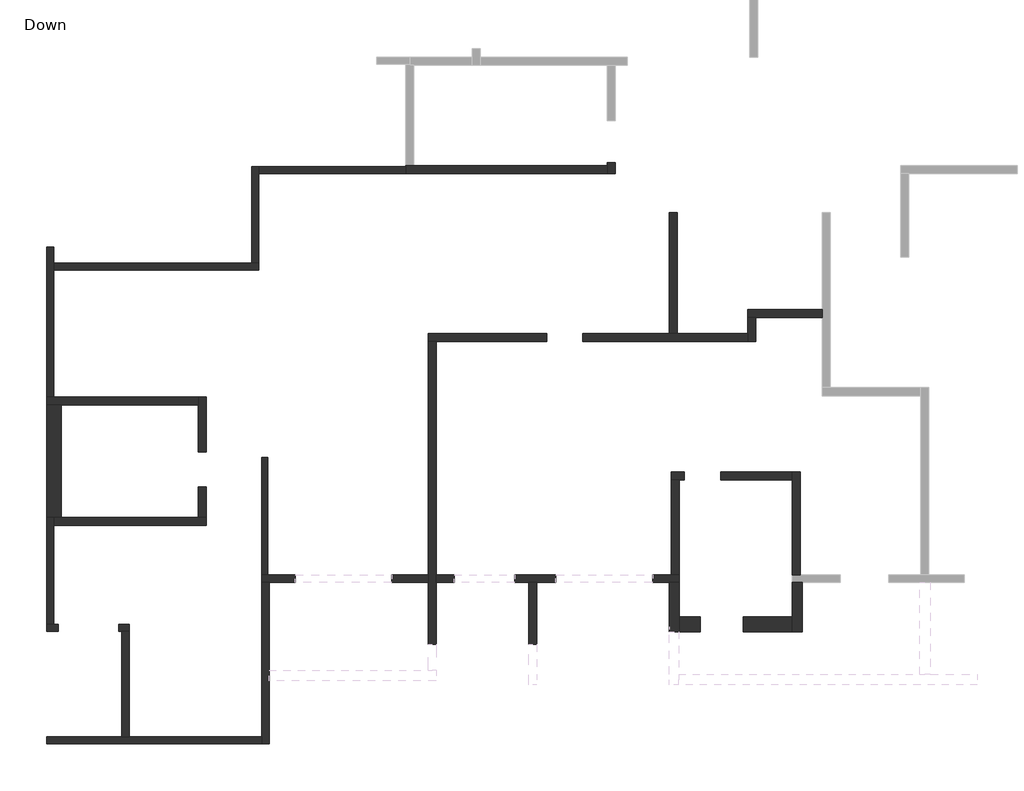
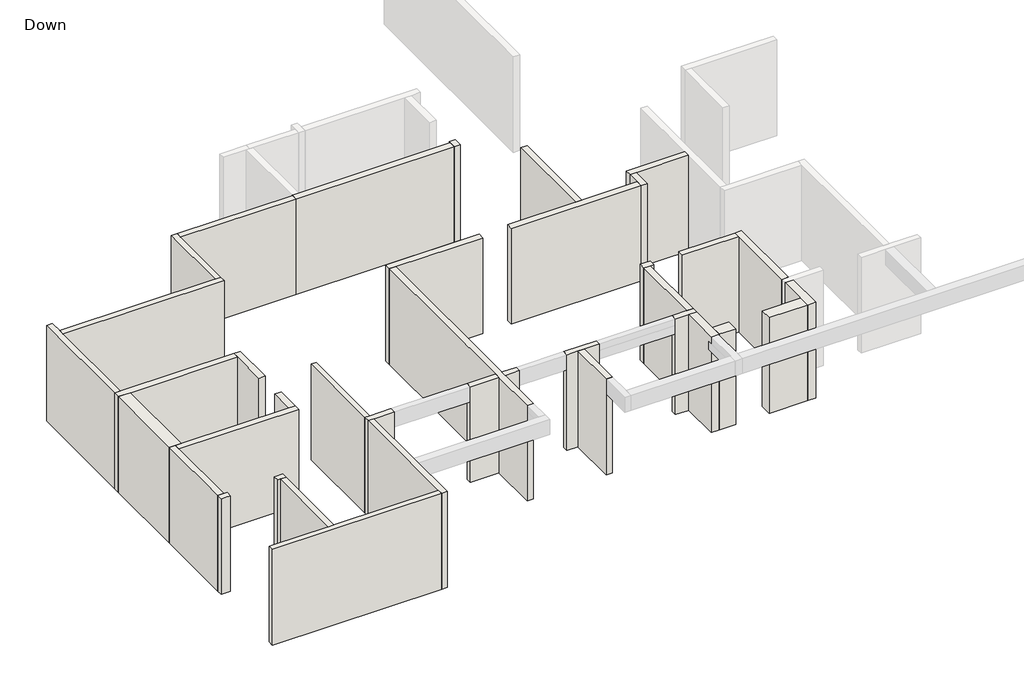
# One storey, part 1 of 3: 38 walls.
"""IFC4 building model written with IfcOpenShell, lengths in millimetres."""

from ifc_helpers import new_model, si_unit, origin, place, context, project, spatial, faceted_brep, element, save

model = new_model("IFC4")

# Units and contexts
model_context = context("Model", 3, world=origin())
ifc_project = project(units=[si_unit("LENGTHUNIT", "METRE", prefix="MILLI")], contexts=[model_context])

# Site, building, storey
site = spatial("IfcSite", under=ifc_project)
building = spatial("IfcBuilding", under=site)
storey = spatial("IfcBuildingStorey", under=building, Name="Down", Elevation=0.0)

# Walls
placement = place(None, origin())
element("IfcWall", 1, ObjectType="15", at=placement, inside=storey, context=model_context, shape_type="Brep", body=[
    faceted_brep([(-13197.6689839, -11344.051338, 0.0), (-13197.6689839, -8414.0928317, 0.0), (-13197.6689839, -8414.0928317, 3000.0), (-13197.6689839, -8414.0928317, 3200.0), (-13197.6689839, -11344.051338, 3200.0), (-13197.6689839, -11344.051338, 3000.0), (-13347.6689839, -11344.051338, 0.0), (-13347.6689839, -11344.051338, 3200.0), (-13347.6689839, -8414.0928317, 3200.0), (-13347.6689839, -8414.0928317, 3000.0), (-13347.6689839, -8414.0928317, 0.0)], [[[0, 1, 2, 3, 4, 5]], [[6, 7, 8, 9, 10]], [[1, 0, 6, 10]], [[3, 2, 1, 10, 9, 8]], [[4, 3, 8, 7]], [[0, 5, 4, 7, 6]]]),
])
element("IfcWall", 2, ObjectType="18", at=placement, inside=storey, context=model_context, shape_type="Brep", body=[
    faceted_brep([(-9216.2167018, -11344.051338, 0.0), (-10116.2830918, -11344.051338, 0.0), (-10116.2830918, -11344.051338, 2700.0), (-10116.2830918, -11344.051338, 3200.0), (-9216.2167018, -11344.051338, 3200.0), (-9216.2167018, -11344.051338, 3000.0), (-9216.2167018, -11524.051338, 0.0), (-9216.2167018, -11524.051338, 2980.0), (-9216.2167018, -11524.051338, 3200.0), (-10116.2830918, -11524.051338, 3200.0), (-10116.2830918, -11524.051338, 2700.0), (-10116.2830918, -11524.051338, 0.0)], [[[0, 1, 2, 3, 4, 5]], [[6, 7, 8, 9, 10, 11]], [[1, 0, 6, 11]], [[3, 2, 1, 11, 10, 9]], [[4, 3, 9, 8]], [[0, 5, 4, 8, 7, 6]]]),
])
element("IfcWall", 3, ObjectType="18", at=placement, inside=storey, context=model_context, shape_type="Brep", body=[
    faceted_brep([(-12517.1627599, -11344.051338, 0.0), (-13197.6689839, -11344.051338, 0.0), (-13347.6689839, -11344.051338, 0.0), (-13347.6689839, -11344.051338, 3200.0), (-13197.6689839, -11344.051338, 3200.0), (-12517.1627599, -11344.051338, 3200.0), (-12517.1627599, -11344.051338, 2700.0), (-12517.1627599, -11524.051338, 0.0), (-12517.1627599, -11524.051338, 2700.0), (-12517.1627599, -11524.051338, 3200.0), (-13167.6689839, -11524.051338, 3200.0), (-13347.6689839, -11524.051338, 3200.0), (-13347.6689839, -11524.051338, 0.0), (-13167.6689839, -11524.051338, 0.0)], [[[0, 1, 2, 3, 4, 5, 6]], [[7, 8, 9, 10, 11, 12, 13]], [[2, 1, 0, 7, 13, 12]], [[5, 4, 3, 11, 10, 9]], [[0, 6, 5, 9, 8, 7]], [[3, 2, 12, 11]]]),
])
element("IfcWall", 4, ObjectType="18", at=placement, inside=storey, context=model_context, shape_type="Brep", body=[
    faceted_brep([(-13347.6689839, -11524.051338, 0.0), (-13347.6689839, -15365.0637861, 0.0), (-13347.6689839, -15545.0637861, 0.0), (-13347.6689839, -15545.0637861, 3200.0), (-13347.6689839, -15365.0637861, 3200.0), (-13347.6689839, -11524.051338, 3200.0), (-13167.6689839, -11524.051338, 0.0), (-13167.6689839, -11524.051338, 2980.0), (-13167.6689839, -11524.051338, 3200.0), (-13167.6689839, -13713.3127488, 3200.0), (-13167.6689839, -15545.0637861, 3200.0), (-13167.6689839, -15545.0637861, 0.0)], [[[0, 1, 2, 3, 4, 5]], [[6, 7, 8, 9, 10, 11]], [[2, 1, 0, 6, 11]], [[5, 4, 3, 10, 9, 8]], [[0, 5, 8, 7, 6]], [[3, 2, 11, 10]]]),
])
element("IfcWall", 5, ObjectType="18", at=placement, inside=storey, context=model_context, shape_type="Brep", body=[
    faceted_brep([(-2966.3411831, -11344.051338, 0.0), (-2966.5901458, -11344.051338, 0.0), (-3166.5901458, -11344.051338, 0.0), (-3636.648237, -11344.051338, 0.0), (-3636.648237, -11344.051338, 2700.0), (-3636.648237, -11344.051338, 3200.0), (-3166.5901458, -11344.051338, 3200.0), (-2966.5901458, -11344.051338, 3200.0), (-2966.3411831, -11344.051338, 3200.0), (-2966.3411831, -11344.051338, 3000.0), (-2966.3411831, -11524.051338, 0.0), (-2966.3411831, -11524.051338, 3200.0), (-3216.3411831, -11524.051338, 3200.0), (-3636.648237, -11524.051338, 3200.0), (-3636.648237, -11524.051338, 2980.0), (-3636.648237, -11524.051338, 2700.0), (-3636.648237, -11524.051338, 0.0), (-3216.3411831, -11524.051338, 0.0), (-3636.648237, -11519.051338, 3200.0)], [[[0, 1, 2, 3, 4, 5, 6, 7, 8, 9]], [[10, 11, 12, 13, 14, 15, 16, 17]], [[3, 2, 1, 0, 10, 17, 16]], [[5, 4, 3, 16, 15, 14, 13, 18]], [[8, 7, 6, 5, 18, 13, 12, 11]], [[0, 9, 8, 11, 10]]]),
])
element("IfcWall", 6, ObjectType="18", at=placement, inside=storey, context=model_context, shape_type="Brep", body=[
    faceted_brep([(-6035.4200213, -11344.051338, 0.0), (-7066.175208, -11344.051338, 0.0), (-7066.175208, -11344.051338, 2700.0), (-7066.175208, -11344.051338, 3200.0), (-6035.4200213, -11344.051338, 3200.0), (-6035.4200213, -11344.051338, 2700.0), (-6035.4200213, -11524.051338, 0.0), (-6035.4200213, -11524.051338, 2700.0), (-6035.4200213, -11524.051338, 2980.0), (-6035.4200213, -11524.051338, 3200.0), (-6516.0175316, -11524.051338, 3200.0), (-6716.0175316, -11524.051338, 3200.0), (-7066.175208, -11524.051338, 3200.0), (-7066.175208, -11524.051338, 2700.0), (-7066.175208, -11524.051338, 0.0), (-6716.0175316, -11524.051338, 0.0), (-6516.0175316, -11524.051338, 0.0), (-6035.4200213, -11519.051338, 3200.0)], [[[0, 1, 2, 3, 4, 5]], [[6, 7, 8, 9, 10, 11, 12, 13, 14, 15, 16]], [[1, 0, 6, 16, 15, 14]], [[3, 2, 1, 14, 13, 12]], [[4, 3, 12, 11, 10, 9, 17]], [[0, 5, 4, 17, 9, 8, 7, 6]]]),
])
element("IfcWall", 7, ObjectType="18", at=placement, inside=storey, context=model_context, shape_type="Brep", body=[
    faceted_brep([(-8566.988486, -11344.051338, 0.0), (-9016.2167018, -11344.051338, 0.0), (-9016.2167018, -11344.051338, 3000.0), (-9016.2167018, -11344.051338, 3200.0), (-8566.988486, -11344.051338, 3200.0), (-8566.988486, -11344.051338, 2700.0), (-8566.988486, -11524.051338, 0.0), (-8566.988486, -11524.051338, 2700.0), (-8566.988486, -11524.051338, 3200.0), (-9016.2167018, -11524.051338, 3200.0), (-9016.2167018, -11524.051338, 0.0)], [[[0, 1, 2, 3, 4, 5]], [[6, 7, 8, 9, 10]], [[1, 0, 6, 10]], [[4, 3, 9, 8]], [[0, 5, 4, 8, 7, 6]], [[3, 2, 1, 10, 9]]]),
])
element("IfcWall", 8, ObjectType="18", at=placement, inside=storey, context=model_context, shape_type="Brep", body=[
    faceted_brep([(-13347.6689839, -15365.0637861, 0.0), (-16646.5071582, -15365.0637861, 0.0), (-16826.5071582, -15365.0637861, 0.0), (-18697.4781126, -15365.0637861, 0.0), (-18697.4781126, -15365.0637861, 3200.0), (-18561.2442958, -15365.0637861, 3200.0), (-16826.5071582, -15365.0637861, 3200.0), (-16646.5071582, -15365.0637861, 3200.0), (-13347.6689839, -15365.0637861, 3200.0), (-13347.6689839, -15365.0637861, 3000.0), (-13347.6689839, -15545.0637861, 0.0), (-13347.6689839, -15545.0637861, 3200.0), (-18697.4781126, -15545.0637861, 3200.0), (-18697.4781126, -15545.0637861, 0.0)], [[[0, 1, 2, 3, 4, 5, 6, 7, 8, 9]], [[10, 11, 12, 13]], [[3, 2, 1, 0, 10, 13]], [[4, 3, 13, 12]], [[8, 7, 6, 5, 4, 12, 11]], [[0, 9, 8, 11, 10]]]),
])
element("IfcWall", 9, ObjectType="18", at=placement, inside=storey, context=model_context, shape_type="Brep", body=[
    faceted_brep([(-16646.5071582, -15365.0637861, 0.0), (-16646.5071582, -12744.5160683, 0.0), (-16646.5071582, -12744.5160683, 3200.0), (-16646.5071582, -15365.0637861, 3200.0), (-16646.5071582, -15365.0637861, 3000.0), (-16826.5071582, -15365.0637861, 0.0), (-16826.5071582, -15365.0637861, 2980.0), (-16826.5071582, -15365.0637861, 3200.0), (-16826.5071582, -12744.5160683, 3200.0), (-16826.5071582, -12744.5160683, 2980.0), (-16826.5071582, -12744.5160683, 0.0)], [[[0, 1, 2, 3, 4]], [[5, 6, 7, 8, 9, 10]], [[1, 0, 5, 10]], [[3, 2, 8, 7]], [[2, 1, 10, 9, 8]], [[0, 4, 3, 7, 6, 5]]]),
])
element("IfcWall", 10, ObjectType="18", at=placement, inside=storey, context=model_context, shape_type="Brep", body=[
    faceted_brep([(-16646.5071582, -12564.5160683, 0.0), (-16907.8847516, -12564.5160683, 0.0), (-16907.8847516, -12564.5160683, 3000.0), (-16907.8847516, -12564.5160683, 3200.0), (-16646.5071582, -12564.5160683, 3200.0), (-16646.5071582, -12564.5160683, 3000.0), (-16646.5071582, -12744.5160683, 0.0), (-16646.5071582, -12744.5160683, 3200.0), (-16826.5071582, -12744.5160683, 3200.0), (-16907.8847516, -12744.5160683, 3200.0), (-16907.8847516, -12744.5160683, 3000.0), (-16907.8847516, -12744.5160683, 0.0), (-16826.5071582, -12744.5160683, 0.0)], [[[0, 1, 2, 3, 4, 5]], [[6, 7, 8, 9, 10, 11, 12]], [[1, 0, 6, 12, 11]], [[3, 2, 1, 11, 10, 9]], [[4, 3, 9, 8, 7]], [[0, 5, 4, 7, 6]]]),
])
element("IfcWall", 11, ObjectType="18", at=placement, inside=storey, context=model_context, shape_type="Brep", body=[
    faceted_brep([(-18406.5901458, -12564.5160683, 0.0), (-18517.4781126, -12564.5160683, 0.0), (-18697.4781126, -12564.5160683, 0.0), (-18697.4781126, -12564.5160683, 3200.0), (-18517.4781126, -12564.5160683, 3200.0), (-18406.5901458, -12564.5160683, 3200.0), (-18406.5901458, -12564.5160683, 3000.0), (-18406.5901458, -12744.5160683, 0.0), (-18406.5901458, -12744.5160683, 3000.0), (-18406.5901458, -12744.5160683, 3200.0), (-18561.2442958, -12744.5160683, 3200.0), (-18697.4781126, -12744.5160683, 3200.0), (-18697.4781126, -12744.5160683, 0.0)], [[[0, 1, 2, 3, 4, 5, 6]], [[7, 8, 9, 10, 11, 12]], [[2, 1, 0, 7, 12]], [[5, 4, 3, 11, 10, 9]], [[0, 6, 5, 9, 8, 7]], [[3, 2, 12, 11]]]),
])
element("IfcWall", 12, ObjectType="18", at=placement, inside=storey, context=model_context, shape_type="Brep", body=[
    faceted_brep([(-18517.4781126, -12564.5160683, 0.0), (-18517.4781126, -10113.0471886, 0.0), (-18517.4781126, -9913.0471886, 0.0), (-18517.4781126, -9913.0471886, 3200.0), (-18517.4781126, -10113.0471886, 3200.0), (-18517.4781126, -12564.5160683, 3200.0), (-18517.4781126, -12564.5160683, 3000.0), (-18697.4781126, -12564.5160683, 0.0), (-18697.4781126, -12564.5160683, 3200.0), (-18697.4781126, -9913.0471886, 3200.0), (-18697.4781126, -9913.0471886, 0.0)], [[[0, 1, 2, 3, 4, 5, 6]], [[7, 8, 9, 10]], [[2, 1, 0, 7, 10]], [[5, 4, 3, 9, 8]], [[0, 6, 5, 8, 7]], [[3, 2, 10, 9]]]),
])
element("IfcWall", 13, ObjectType="18", at=placement, inside=storey, context=model_context, shape_type="Brep", body=[
    faceted_brep([(-18517.4781126, -6913.2795537, 0.0), (-18517.4781126, -3764.1011305, 0.0), (-18517.4781126, -3584.1011305, 0.0), (-18517.4781126, -3184.4330807, 0.0), (-18517.4781126, -3184.4330807, 3200.0), (-18517.4781126, -3584.1011305, 3200.0), (-18517.4781126, -3764.1011305, 3200.0), (-18517.4781126, -6913.2795537, 3200.0), (-18517.4781126, -6913.2795537, 3000.0), (-18697.4781126, -6913.2795537, 0.0), (-18697.4781126, -6913.2795537, 3200.0), (-18697.4781126, -3184.4330807, 3200.0), (-18697.4781126, -3184.4330807, 0.0)], [[[0, 1, 2, 3, 4, 5, 6, 7, 8]], [[9, 10, 11, 12]], [[3, 2, 1, 0, 9, 12]], [[4, 3, 12, 11]], [[7, 6, 5, 4, 11, 10]], [[0, 8, 7, 10, 9]]]),
])
element("IfcWall", 14, ObjectType="18", at=placement, inside=storey, context=model_context, shape_type="Brep", body=[
    faceted_brep([(-18517.4781126, -3764.1011305, 0.0), (-13417.2291499, -3764.1011305, 0.0), (-13417.2291499, -3764.1011305, 3000.0), (-13417.2291499, -3764.1011305, 3200.0), (-18517.4781126, -3764.1011305, 3200.0), (-18517.4781126, -3764.1011305, 3000.0), (-18517.4781126, -3584.1011305, 0.0), (-18517.4781126, -3584.1011305, 3200.0), (-13597.2291499, -3584.1011305, 3200.0), (-13417.2291499, -3584.1011305, 3200.0), (-13417.2291499, -3584.1011305, 0.0), (-13597.2291499, -3584.1011305, 0.0)], [[[0, 1, 2, 3, 4, 5]], [[6, 7, 8, 9, 10, 11]], [[1, 0, 6, 11, 10]], [[4, 3, 9, 8, 7]], [[0, 5, 4, 7, 6]], [[3, 2, 1, 10, 9]]]),
])
element("IfcWall", 15, ObjectType="18", at=placement, inside=storey, context=model_context, shape_type="Brep", body=[
    faceted_brep([(-13417.2291499, -3584.1011305, 0.0), (-13417.2291499, -1364.051338, 0.0), (-13417.2291499, -1184.051338, 0.0), (-13417.2291499, -1184.051338, 3200.0), (-13417.2291499, -1364.051338, 3200.0), (-13417.2291499, -3584.1011305, 3200.0), (-13597.2291499, -3584.1011305, 0.0), (-13597.2291499, -3584.1011305, 3200.0), (-13597.2291499, -1184.051338, 3200.0), (-13597.2291499, -1184.051338, 0.0)], [[[0, 1, 2, 3, 4, 5]], [[6, 7, 8, 9]], [[2, 1, 0, 6, 9]], [[5, 4, 3, 8, 7]], [[0, 5, 7, 6]], [[3, 2, 9, 8]]]),
])
element("IfcWall", 16, ObjectType="18", at=placement, inside=storey, context=model_context, shape_type="Brep", body=[
    faceted_brep([(-13417.2291499, -1364.051338, 0.0), (-9767.2291499, -1364.051338, 0.0), (-9767.2291499, -1364.051338, 3200.0), (-13417.2291499, -1364.051338, 3200.0), (-13417.2291499, -1364.051338, 3000.0), (-13417.2291499, -1184.051338, 0.0), (-13417.2291499, -1184.051338, 3200.0), (-9767.2291499, -1184.051338, 3200.0), (-9767.2291499, -1184.051338, 0.0)], [[[0, 1, 2, 3, 4]], [[5, 6, 7, 8]], [[1, 0, 5, 8]], [[2, 1, 8, 7]], [[3, 2, 7, 6]], [[0, 4, 3, 6, 5]]]),
])
element("IfcWall", 17, ObjectType="20", at=placement, inside=storey, context=model_context, shape_type="Brep", body=[
    faceted_brep([(35.0364103, -11344.051338, 0.0), (35.0364103, -8782.9724998, 0.0), (35.0364103, -8782.9724998, 3000.0), (35.0364103, -8782.9724998, 3200.0), (35.0364103, -11344.051338, 3200.0), (35.0364103, -11344.051338, 3000.0), (-164.9635897, -11344.051338, 0.0), (-164.9635897, -11344.051338, 3200.0), (-164.9635897, -8982.9724998, 3200.0), (-164.9635897, -8782.9724998, 3200.0), (-164.9635897, -8782.9724998, 0.0), (-164.9635897, -8982.9724998, 0.0)], [[[0, 1, 2, 3, 4, 5]], [[6, 7, 8, 9, 10, 11]], [[1, 0, 6, 11, 10]], [[4, 3, 9, 8, 7]], [[0, 5, 4, 7, 6]], [[3, 2, 1, 10, 9]]]),
])
element("IfcWall", 18, ObjectType="20", at=placement, inside=storey, context=model_context, shape_type="Brep", body=[
    faceted_brep([(-164.9635897, -8782.9724998, 0.0), (-1944.0175316, -8782.9724998, 0.0), (-1944.0175316, -8782.9724998, 3000.0), (-1944.0175316, -8782.9724998, 3200.0), (-164.9635897, -8782.9724998, 3200.0), (-164.9635897, -8982.9724998, 0.0), (-164.9635897, -8982.9724998, 3000.0), (-164.9635897, -8982.9724998, 3200.0), (-1944.0175316, -8982.9724998, 3200.0), (-1944.0175316, -8982.9724998, 3000.0), (-1944.0175316, -8982.9724998, 0.0)], [[[0, 1, 2, 3, 4]], [[5, 6, 7, 8, 9, 10]], [[1, 0, 5, 10]], [[3, 2, 1, 10, 9, 8]], [[4, 3, 8, 7]], [[0, 4, 7, 6, 5]]]),
])
element("IfcWall", 19, ObjectType="20", at=placement, inside=storey, context=model_context, shape_type="Brep", body=[
    faceted_brep([(-2850.4075731, -8782.9724998, 0.0), (-3166.5901458, -8782.9724998, 0.0), (-3166.5901458, -8782.9724998, 3000.0), (-3166.5901458, -8782.9724998, 3200.0), (-2850.4075731, -8782.9724998, 3200.0), (-2850.4075731, -8782.9724998, 3000.0), (-2850.4075731, -8982.9724998, 0.0), (-2850.4075731, -8982.9724998, 3000.0), (-2850.4075731, -8982.9724998, 3200.0), (-2966.5901458, -8982.9724998, 3200.0), (-3166.5901458, -8982.9724998, 3200.0), (-3166.5901458, -8982.9724998, 0.0), (-2966.5901458, -8982.9724998, 0.0)], [[[0, 1, 2, 3, 4, 5]], [[6, 7, 8, 9, 10, 11, 12]], [[1, 0, 6, 12, 11]], [[4, 3, 10, 9, 8]], [[0, 5, 4, 8, 7, 6]], [[3, 2, 1, 11, 10]]]),
])
element("IfcWall", 20, ObjectType="20", at=placement, inside=storey, context=model_context, shape_type="Brep", body=[
    faceted_brep([(-3166.5901458, -8982.9724998, 0.0), (-3166.5901458, -11344.051338, 0.0), (-3166.5901458, -11344.051338, 3000.0), (-3166.5901458, -11344.051338, 3200.0), (-3166.5901458, -8982.9724998, 3200.0), (-2966.5901458, -8982.9724998, 0.0), (-2966.5901458, -8982.9724998, 3000.0), (-2966.5901458, -8982.9724998, 3200.0), (-2966.5901458, -11344.051338, 3200.0), (-2966.5901458, -11344.051338, 3000.0), (-2966.5901458, -11344.051338, 0.0)], [[[0, 1, 2, 3, 4]], [[5, 6, 7, 8, 9, 10]], [[1, 0, 5, 10]], [[4, 3, 8, 7]], [[0, 4, 7, 6, 5]], [[3, 2, 1, 10, 9, 8]]]),
])
element("IfcWall", 21, ObjectType="20", at=placement, inside=storey, context=model_context, shape_type="Brep", body=[
    faceted_brep([(583.3351654, -4733.7276865, 0.0), (-1265.2789424, -4733.7276865, 0.0), (-1265.2789424, -4733.7276865, 3200.0), (583.3351654, -4733.7276865, 3200.0), (583.3351654, -4933.7276865, 0.0), (583.3351654, -4933.7276865, 3000.0), (583.3351654, -4933.7276865, 3200.0), (-1065.2789424, -4933.7276865, 3200.0), (-1265.2789424, -4933.7276865, 3200.0), (-1265.2789424, -4933.7276865, 0.0), (-1065.2789424, -4933.7276865, 0.0)], [[[0, 1, 2, 3]], [[4, 5, 6, 7, 8, 9, 10]], [[1, 0, 4, 10, 9]], [[3, 2, 8, 7, 6]], [[0, 3, 6, 5, 4]], [[2, 1, 9, 8]]]),
])
element("IfcWall", 22, ObjectType="20", at=placement, inside=storey, context=model_context, shape_type="Brep", body=[
    faceted_brep([(-1265.2789424, -4933.7276865, 0.0), (-1265.2789424, -5334.7235371, 0.0), (-1265.2789424, -5534.7235371, 0.0), (-1265.2789424, -5534.7235371, 3200.0), (-1265.2789424, -5334.7235371, 3200.0), (-1265.2789424, -4933.7276865, 3200.0), (-1065.2789424, -4933.7276865, 0.0), (-1065.2789424, -4933.7276865, 3000.0), (-1065.2789424, -4933.7276865, 3200.0), (-1065.2789424, -5534.7235371, 3200.0), (-1065.2789424, -5534.7235371, 3000.0), (-1065.2789424, -5534.7235371, 0.0)], [[[0, 1, 2, 3, 4, 5]], [[6, 7, 8, 9, 10, 11]], [[2, 1, 0, 6, 11]], [[5, 4, 3, 9, 8]], [[0, 5, 8, 7, 6]], [[3, 2, 11, 10, 9]]]),
])
element("IfcWall", 23, ObjectType="20", at=placement, inside=storey, context=model_context, shape_type="Brep", body=[
    faceted_brep([(-1265.2789424, -5334.7235371, 0.0), (-3016.9303947, -5334.7235371, 0.0), (-3216.9303947, -5334.7235371, 0.0), (-5367.2208511, -5334.7235371, 0.0), (-5367.2208511, -5334.7235371, 3000.0), (-5367.2208511, -5334.7235371, 3200.0), (-3216.9303947, -5334.7235371, 3200.0), (-3016.9303947, -5334.7235371, 3200.0), (-1265.2789424, -5334.7235371, 3200.0), (-1265.2789424, -5534.7235371, 0.0), (-1265.2789424, -5534.7235371, 3200.0), (-5367.2208511, -5534.7235371, 3200.0), (-5367.2208511, -5534.7235371, 3000.0), (-5367.2208511, -5534.7235371, 0.0)], [[[0, 1, 2, 3, 4, 5, 6, 7, 8]], [[9, 10, 11, 12, 13]], [[3, 2, 1, 0, 9, 13]], [[5, 4, 3, 13, 12, 11]], [[8, 7, 6, 5, 11, 10]], [[0, 8, 10, 9]]]),
])
element("IfcWall", 24, ObjectType="20", at=placement, inside=storey, context=model_context, shape_type="Brep", body=[
    faceted_brep([(-6267.2872412, -5334.7235371, 0.0), (-9216.2167018, -5334.7235371, 0.0), (-9216.2167018, -5334.7235371, 3000.0), (-9216.2167018, -5334.7235371, 3200.0), (-6267.2872412, -5334.7235371, 3200.0), (-6267.2872412, -5334.7235371, 3000.0), (-6267.2872412, -5534.7235371, 0.0), (-6267.2872412, -5534.7235371, 3000.0), (-6267.2872412, -5534.7235371, 3200.0), (-9016.2167018, -5534.7235371, 3200.0), (-9216.2167018, -5534.7235371, 3200.0), (-9216.2167018, -5534.7235371, 0.0), (-9016.2167018, -5534.7235371, 0.0)], [[[0, 1, 2, 3, 4, 5]], [[6, 7, 8, 9, 10, 11, 12]], [[1, 0, 6, 12, 11]], [[4, 3, 10, 9, 8]], [[0, 5, 4, 8, 7, 6]], [[3, 2, 1, 11, 10]]]),
])
element("IfcWall", 25, ObjectType="20", at=placement, inside=storey, context=model_context, shape_type="Brep", body=[
    faceted_brep([(-3216.9303947, -2332.8480185, 0.0), (-3216.9303947, -5334.7235371, 0.0), (-3216.9303947, -5334.7235371, 3000.0), (-3216.9303947, -5334.7235371, 3200.0), (-3216.9303947, -2332.8480185, 3200.0), (-3216.9303947, -2332.8480185, 3000.0), (-3016.9303947, -2332.8480185, 0.0), (-3016.9303947, -2332.8480185, 3200.0), (-3016.9303947, -5334.7235371, 3200.0), (-3016.9303947, -5334.7235371, 0.0)], [[[0, 1, 2, 3, 4, 5]], [[6, 7, 8, 9]], [[1, 0, 6, 9]], [[4, 3, 8, 7]], [[0, 5, 4, 7, 6]], [[3, 2, 1, 9, 8]]]),
])
element("IfcWall", 26, ObjectType="20", at=placement, inside=storey, context=model_context, shape_type="Brep", body=[
    faceted_brep([(-9216.2167018, -5534.7235371, 0.0), (-9216.2167018, -11344.051338, 0.0), (-9216.2167018, -11524.051338, 0.0), (-9216.2167018, -13068.3003006, 0.0), (-9216.2167018, -13068.3003006, 2700.0), (-9216.2167018, -13068.3003006, 2980.0), (-9216.2167018, -13068.3003006, 3200.0), (-9216.2167018, -11524.051338, 3200.0), (-9216.2167018, -11344.051338, 3200.0), (-9216.2167018, -5534.7235371, 3200.0), (-9016.2167018, -5534.7235371, 0.0), (-9016.2167018, -5534.7235371, 3000.0), (-9016.2167018, -5534.7235371, 3200.0), (-9016.2167018, -11344.051338, 3200.0), (-9016.2167018, -11524.051338, 3200.0), (-9016.2167018, -13068.3003006, 3200.0), (-9016.2167018, -13068.3003006, 2700.0), (-9016.2167018, -13068.3003006, 0.0), (-9016.2167018, -11524.051338, 0.0), (-9016.2167018, -11344.051338, 0.0), (-9211.2167018, -13068.3003006, 3200.0)], [[[0, 1, 2, 3, 4, 5, 6, 7, 8, 9]], [[10, 11, 12, 13, 14, 15, 16, 17, 18, 19]], [[3, 2, 1, 0, 10, 19, 18, 17]], [[6, 5, 4, 3, 17, 16, 15, 20]], [[9, 8, 7, 6, 20, 15, 14, 13, 12]], [[0, 9, 12, 11, 10]]]),
])
element("IfcWall", 27, ObjectType="20", at=placement, inside=storey, context=model_context, shape_type="Brep", body=[
    faceted_brep([(-6716.0175316, -11524.051338, 0.0), (-6716.0175316, -13068.3003006, 0.0), (-6716.0175316, -13068.3003006, 2700.0), (-6716.0175316, -13068.3003006, 3200.0), (-6716.0175316, -11524.051338, 3200.0), (-6516.0175316, -11524.051338, 0.0), (-6516.0175316, -11524.051338, 2980.0), (-6516.0175316, -11524.051338, 3200.0), (-6516.0175316, -13068.3003006, 3200.0), (-6516.0175316, -13068.3003006, 2700.0), (-6516.0175316, -13068.3003006, 0.0)], [[[0, 1, 2, 3, 4]], [[5, 6, 7, 8, 9, 10]], [[1, 0, 5, 10]], [[3, 2, 1, 10, 9, 8]], [[4, 3, 8, 7]], [[0, 4, 7, 6, 5]]]),
])
element("IfcWall", 28, ObjectType="20", at=placement, inside=storey, context=model_context, shape_type="Brep", body=[
    faceted_brep([(-18517.4781126, -10113.0471886, 0.0), (-14726.2250005, -10113.0471886, 0.0), (-14726.2250005, -10113.0471886, 3000.0), (-14726.2250005, -10113.0471886, 3200.0), (-18517.4781126, -10113.0471886, 3200.0), (-18517.4781126, -10113.0471886, 3000.0), (-18517.4781126, -9913.0471886, 0.0), (-18517.4781126, -9913.0471886, 3200.0), (-18327.4781126, -9913.0471886, 3200.0), (-14926.2250005, -9913.0471886, 3200.0), (-14726.2250005, -9913.0471886, 3200.0), (-14726.2250005, -9913.0471886, 0.0), (-14926.2250005, -9913.0471886, 0.0), (-18327.4781126, -9913.0471886, 0.0)], [[[0, 1, 2, 3, 4, 5]], [[6, 7, 8, 9, 10, 11, 12, 13]], [[1, 0, 6, 13, 12, 11]], [[4, 3, 10, 9, 8, 7]], [[0, 5, 4, 7, 6]], [[3, 2, 1, 11, 10]]]),
])
element("IfcWall", 29, ObjectType="20", at=placement, inside=storey, context=model_context, shape_type="Brep", body=[
    faceted_brep([(-14726.2250005, -9913.0471886, 0.0), (-14726.2250005, -9149.744284, 0.0), (-14726.2250005, -9149.744284, 3000.0), (-14726.2250005, -9149.744284, 3200.0), (-14726.2250005, -9913.0471886, 3200.0), (-14926.2250005, -9913.0471886, 0.0), (-14926.2250005, -9913.0471886, 3000.0), (-14926.2250005, -9913.0471886, 3200.0), (-14926.2250005, -9149.744284, 3200.0), (-14926.2250005, -9149.744284, 3000.0), (-14926.2250005, -9149.744284, 0.0)], [[[0, 1, 2, 3, 4]], [[5, 6, 7, 8, 9, 10]], [[1, 0, 5, 10]], [[3, 2, 1, 10, 9, 8]], [[4, 3, 8, 7]], [[0, 4, 7, 6, 5]]]),
])
element("IfcWall", 30, ObjectType="20", at=placement, inside=storey, context=model_context, shape_type="Brep", body=[
    faceted_brep([(-14726.2250005, -8279.1882674, 0.0), (-14726.2250005, -6913.2795537, 0.0), (-14726.2250005, -6913.2795537, 3000.0), (-14726.2250005, -6913.2795537, 3200.0), (-14726.2250005, -8279.1882674, 3200.0), (-14726.2250005, -8279.1882674, 3000.0), (-14926.2250005, -8279.1882674, 0.0), (-14926.2250005, -8279.1882674, 3000.0), (-14926.2250005, -8279.1882674, 3200.0), (-14926.2250005, -7113.2795537, 3200.0), (-14926.2250005, -6913.2795537, 3200.0), (-14926.2250005, -6913.2795537, 0.0), (-14926.2250005, -7113.2795537, 0.0)], [[[0, 1, 2, 3, 4, 5]], [[6, 7, 8, 9, 10, 11, 12]], [[1, 0, 6, 12, 11]], [[4, 3, 10, 9, 8]], [[0, 5, 4, 8, 7, 6]], [[3, 2, 1, 11, 10]]]),
])
element("IfcWall", 31, ObjectType="20", at=placement, inside=storey, context=model_context, shape_type="Brep", body=[
    faceted_brep([(-14926.2250005, -6913.2795537, 0.0), (-18517.4781126, -6913.2795537, 0.0), (-18697.4781126, -6913.2795537, 0.0), (-18697.4781126, -6913.2795537, 3200.0), (-18517.4781126, -6913.2795537, 3200.0), (-14926.2250005, -6913.2795537, 3200.0), (-14926.2250005, -7113.2795537, 0.0), (-14926.2250005, -7113.2795537, 3000.0), (-14926.2250005, -7113.2795537, 3200.0), (-18327.4781126, -7113.2795537, 3200.0), (-18697.4781126, -7113.2795537, 3200.0), (-18697.4781126, -7113.2795537, 0.0), (-18327.4781126, -7113.2795537, 0.0)], [[[0, 1, 2, 3, 4, 5]], [[6, 7, 8, 9, 10, 11, 12]], [[2, 1, 0, 6, 12, 11]], [[5, 4, 3, 10, 9, 8]], [[0, 5, 8, 7, 6]], [[3, 2, 11, 10]]]),
])
element("IfcWall", 32, ObjectType="20", at=placement, inside=storey, context=model_context, shape_type="Brep", body=[
    faceted_brep([(-9767.2291499, -1364.051338, 0.0), (-4766.2250005, -1364.051338, 0.0), (-4766.2250005, -1364.051338, 3200.0), (-9767.2291499, -1364.051338, 3200.0), (-9767.2291499, -1164.051338, 0.0), (-9767.2291499, -1164.051338, 3200.0), (-9766.1254155, -1164.051338, 3200.0), (-9566.1254155, -1164.051338, 3200.0), (-4766.2250005, -1164.051338, 3200.0), (-4766.2250005, -1164.051338, 0.0), (-9566.1254155, -1164.051338, 0.0), (-9766.1254155, -1164.051338, 0.0), (-9767.2291499, -1184.051338, 0.0), (-9767.2291499, -1184.051338, 3200.0)], [[[0, 1, 2, 3]], [[4, 5, 6, 7, 8, 9, 10, 11]], [[1, 0, 12, 4, 11, 10, 9]], [[3, 2, 8, 7, 6, 5, 13]], [[0, 3, 13, 5, 4, 12]], [[2, 1, 9, 8]]]),
])
element("IfcWall", 33, ObjectType="20", at=placement, inside=storey, context=model_context, shape_type="Brep", body=[
    faceted_brep([(-4566.2250005, -1364.051338, 0.0), (-4566.2250005, -1089.1965662, 0.0), (-4566.2250005, -1089.1965662, 3200.0), (-4566.2250005, -1364.051338, 3200.0), (-4566.2250005, -1364.051338, 3000.0), (-4766.2250005, -1364.051338, 0.0), (-4766.2250005, -1364.051338, 3200.0), (-4766.2250005, -1164.051338, 3200.0), (-4766.2250005, -1089.1965662, 3200.0), (-4766.2250005, -1089.1965662, 0.0), (-4766.2250005, -1164.051338, 0.0)], [[[0, 1, 2, 3, 4]], [[5, 6, 7, 8, 9, 10]], [[1, 0, 5, 10, 9]], [[2, 1, 9, 8]], [[3, 2, 8, 7, 6]], [[0, 4, 3, 6, 5]]]),
])
element("IfcWall", 34, ObjectType="25", at=placement, inside=storey, context=model_context, shape_type="Brep", body=[
    faceted_brep([(-3216.3411831, -11524.051338, 0.0), (-3216.3411831, -12754.2256118, 0.0), (-3216.3411831, -12754.2256118, 2700.0), (-3216.3411831, -12754.2256118, 2980.0), (-3216.3411831, -12754.2256118, 3200.0), (-3216.3411831, -11524.051338, 3200.0), (-3216.3411831, -11524.051338, 2980.0), (-2966.3411831, -11524.051338, 0.0), (-2966.3411831, -11524.051338, 3200.0), (-2966.3411831, -12384.2256118, 3200.0), (-2966.3411831, -12754.2256118, 3200.0), (-2966.3411831, -12754.2256118, 0.0), (-2966.3411831, -12384.2256118, 0.0), (-3211.3411831, -12754.2256118, 3200.0), (-2990.4458666, -12754.2256118, 3200.0)], [[[0, 1, 2, 3, 4, 5, 6]], [[7, 8, 9, 10, 11, 12]], [[1, 0, 7, 12, 11]], [[5, 4, 13, 14, 10, 9, 8]], [[0, 6, 5, 8, 7]], [[4, 3, 2, 1, 11, 10, 14, 13]]]),
])
element("IfcWall", 35, ObjectType="25", at=placement, inside=storey, context=model_context, shape_type="Brep", body=[
    faceted_brep([(-164.9635897, -11524.051338, 0.0), (-164.9635897, -12384.2256118, 0.0), (-164.9635897, -12754.2256118, 0.0), (-164.9635897, -12754.2256118, 3200.0), (-164.9635897, -12384.2256118, 3200.0), (-164.9635897, -11524.051338, 3200.0), (85.0364103, -11524.051338, 0.0), (85.0364103, -11524.051338, 3200.0), (85.0364103, -12754.2256118, 3200.0), (85.0364103, -12754.2256118, 0.0)], [[[0, 1, 2, 3, 4, 5]], [[6, 7, 8, 9]], [[2, 1, 0, 6, 9]], [[5, 4, 3, 8, 7]], [[0, 5, 7, 6]], [[3, 2, 9, 8]]]),
])
element("IfcWall", 36, ObjectType="37", at=placement, inside=storey, context=model_context, shape_type="Brep", body=[
    faceted_brep([(-2966.3411831, -12754.2256118, 0.0), (-2445.6938802, -12754.2256118, 0.0), (-2445.6938802, -12754.2256118, 3200.0), (-2966.3411831, -12754.2256118, 3200.0), (-2966.3411831, -12384.2256118, 0.0), (-2966.3411831, -12384.2256118, 3000.0), (-2966.3411831, -12384.2256118, 3200.0), (-2445.6938802, -12384.2256118, 3200.0), (-2445.6938802, -12384.2256118, 0.0)], [[[0, 1, 2, 3]], [[4, 5, 6, 7, 8]], [[1, 0, 4, 8]], [[2, 1, 8, 7]], [[3, 2, 7, 6]], [[0, 3, 6, 5, 4]]]),
])
element("IfcWall", 37, ObjectType="37", at=placement, inside=storey, context=model_context, shape_type="Brep", body=[
    faceted_brep([(-1385.42832, -12754.2256118, 0.0), (-164.9635897, -12754.2256118, 0.0), (-164.9635897, -12754.2256118, 3200.0), (-1385.42832, -12754.2256118, 3200.0), (-1385.42832, -12384.2256118, 0.0), (-1385.42832, -12384.2256118, 3200.0), (-164.9635897, -12384.2256118, 3200.0), (-164.9635897, -12384.2256118, 3000.0), (-164.9635897, -12384.2256118, 0.0)], [[[0, 1, 2, 3]], [[4, 5, 6, 7, 8]], [[1, 0, 4, 8]], [[3, 2, 6, 5]], [[0, 3, 5, 4]], [[2, 1, 8, 7, 6]]]),
])
element("IfcWall", 38, ObjectType="37", at=placement, inside=storey, context=model_context, shape_type="Brep", body=[
    faceted_brep([(-18327.4781126, -9913.0471886, 0.0), (-18327.4781126, -7113.2795537, 0.0), (-18327.4781126, -7113.2795537, 3000.0), (-18327.4781126, -7113.2795537, 3200.0), (-18327.4781126, -9913.0471886, 3200.0), (-18327.4781126, -9913.0471886, 3000.0), (-18697.4781126, -9913.0471886, 0.0), (-18697.4781126, -9913.0471886, 3200.0), (-18697.4781126, -7113.2795537, 3200.0), (-18697.4781126, -7113.2795537, 0.0), (-18517.4781126, -9913.0471886, 0.0), (-18517.4781126, -9913.0471886, 3200.0)], [[[0, 1, 2, 3, 4, 5]], [[6, 7, 8, 9]], [[1, 0, 10, 6, 9]], [[4, 3, 8, 7, 11]], [[0, 5, 4, 11, 7, 6, 10]], [[3, 2, 1, 9, 8]]]),
])

save(model, "model.ifc")

# Revit data of these elements
# Project information
#   Project Issue Date = "Issue Date"
#   Project Status = "Project Status"
#   Client Name = "לקוח"
#   Project Address = "Enter address here"
#   Project Name = "Project 032"
#   Project Number = "מספר פרויקט"
# Type "15"
#   Layers, outside or top first: 15 cm "Concrete" (function 1)
# Type "18"
#   Layers, outside or top first: 18 cm "Concrete" (function 1)
# Type "20"
#   Layers, outside or top first: 20 cm "Concrete" (function 1)
# Type "25"
#   Layers, outside or top first: 25 cm "Concrete" (function 1)
# Type "37"
#   Layers, outside or top first: 37 cm "Concrete" (function 1)
# Element 1 (IfcWall, "15")
#   Comments = ""
#   Mark = "W100"
#   SOFiSTiK_EdgeZones = "W101"
#   SOFiSTiK_AMG_Comments = ""
#   Top Offset = 0 cm
#   Base Offset = 0 cm
#   wall height = 320 cm
#   SOFiSTiK_AMG_Scheduled = yes
#   SOFiSTiK_AMG_Adjusted = yes
#   Phase Created = New Construction
#   Base Constraint = Down
#   Top Constraint = Typical Floor
#   Materials on its faces: "Concrete"
# Element 2 (IfcWall, "18")
#   Comments = ""
#   Mark = "W69"
#   SOFiSTiK_EdgeZones = "W70"
#   SOFiSTiK_AMG_Comments = ""
#   Top Offset = 0 cm
#   Base Offset = 0 cm
#   wall height = 320 cm
#   SOFiSTiK_AMG_Scheduled = yes
#   SOFiSTiK_AMG_Adjusted = yes
#   Phase Created = New Construction
#   Base Constraint = Down
#   Top Constraint = Typical Floor
#   Materials on its faces: "Concrete"
# Element 3 (IfcWall, "18")
#   Comments = ""
#   Mark = "W70"
#   SOFiSTiK_EdgeZones = "W71"
#   SOFiSTiK_AMG_Comments = ""
#   Top Offset = 0 cm
#   Base Offset = 0 cm
#   wall height = 320 cm
#   SOFiSTiK_AMG_Scheduled = yes
#   SOFiSTiK_AMG_Adjusted = yes
#   Phase Created = New Construction
#   Base Constraint = Down
#   Top Constraint = Typical Floor
#   Materials on its faces: "Concrete"
# Element 4 (IfcWall, "18")
#   Comments = ""
#   Mark = "W71"
#   SOFiSTiK_EdgeZones = "W72"
#   SOFiSTiK_AMG_Comments = ""
#   Top Offset = 0 cm
#   Base Offset = 0 cm
#   wall height = 320 cm
#   SOFiSTiK_AMG_Scheduled = yes
#   SOFiSTiK_AMG_Adjusted = yes
#   Phase Created = New Construction
#   Base Constraint = Down
#   Top Constraint = Typical Floor
#   Materials on its faces: "Concrete"
# Element 5 (IfcWall, "18")
#   Comments = ""
#   Mark = "W72"
#   SOFiSTiK_EdgeZones = "W73"
#   SOFiSTiK_AMG_Comments = ""
#   Top Offset = 0 cm
#   Base Offset = 0 cm
#   wall height = 320 cm
#   SOFiSTiK_AMG_Scheduled = yes
#   SOFiSTiK_AMG_Adjusted = yes
#   Phase Created = New Construction
#   Base Constraint = Down
#   Top Constraint = Typical Floor
#   Materials on its faces: "Concrete"
# Element 6 (IfcWall, "18")
#   Comments = ""
#   Mark = "W73"
#   SOFiSTiK_EdgeZones = "W74"
#   SOFiSTiK_AMG_Comments = ""
#   Top Offset = 0 cm
#   Base Offset = 0 cm
#   wall height = 320 cm
#   SOFiSTiK_AMG_Scheduled = yes
#   SOFiSTiK_AMG_Adjusted = yes
#   Phase Created = New Construction
#   Base Constraint = Down
#   Top Constraint = Typical Floor
#   Materials on its faces: "Concrete"
# Element 7 (IfcWall, "18")
#   Comments = ""
#   Mark = "W74"
#   SOFiSTiK_EdgeZones = "W75"
#   SOFiSTiK_AMG_Comments = ""
#   Top Offset = 0 cm
#   Base Offset = 0 cm
#   wall height = 320 cm
#   SOFiSTiK_AMG_Scheduled = yes
#   SOFiSTiK_AMG_Adjusted = yes
#   Phase Created = New Construction
#   Base Constraint = Down
#   Top Constraint = Typical Floor
#   Materials on its faces: "Concrete"
# Element 8 (IfcWall, "18")
#   Comments = ""
#   Mark = "W75"
#   SOFiSTiK_EdgeZones = "W76"
#   SOFiSTiK_AMG_Comments = ""
#   Top Offset = 0 cm
#   Base Offset = 0 cm
#   wall height = 320 cm
#   SOFiSTiK_AMG_Scheduled = yes
#   SOFiSTiK_AMG_Adjusted = yes
#   Phase Created = New Construction
#   Base Constraint = Down
#   Top Constraint = Typical Floor
#   Materials on its faces: "Concrete"
# Element 9 (IfcWall, "18")
#   Comments = ""
#   Mark = "W76"
#   SOFiSTiK_EdgeZones = "W77"
#   SOFiSTiK_AMG_Comments = ""
#   Top Offset = 0 cm
#   Base Offset = 0 cm
#   wall height = 320 cm
#   SOFiSTiK_AMG_Scheduled = yes
#   SOFiSTiK_AMG_Adjusted = yes
#   Phase Created = New Construction
#   Base Constraint = Down
#   Top Constraint = Typical Floor
#   Materials on its faces: "Concrete"
# Element 10 (IfcWall, "18")
#   Comments = ""
#   Mark = "W77"
#   SOFiSTiK_EdgeZones = "W78"
#   SOFiSTiK_AMG_Comments = ""
#   Top Offset = 0 cm
#   Base Offset = 0 cm
#   wall height = 320 cm
#   SOFiSTiK_AMG_Scheduled = yes
#   SOFiSTiK_AMG_Adjusted = yes
#   Phase Created = New Construction
#   Base Constraint = Down
#   Top Constraint = Typical Floor
#   Materials on its faces: "Concrete"
# Element 11 (IfcWall, "18")
#   Comments = ""
#   Mark = "W78"
#   SOFiSTiK_EdgeZones = "W79"
#   SOFiSTiK_AMG_Comments = ""
#   Top Offset = 0 cm
#   Base Offset = 0 cm
#   wall height = 320 cm
#   SOFiSTiK_AMG_Scheduled = yes
#   SOFiSTiK_AMG_Adjusted = yes
#   Phase Created = New Construction
#   Base Constraint = Down
#   Top Constraint = Typical Floor
#   Materials on its faces: "Concrete"
# Element 12 (IfcWall, "18")
#   Comments = ""
#   Mark = "W79"
#   SOFiSTiK_EdgeZones = "W80"
#   SOFiSTiK_AMG_Comments = ""
#   Top Offset = 0 cm
#   Base Offset = 0 cm
#   wall height = 320 cm
#   SOFiSTiK_AMG_Scheduled = yes
#   SOFiSTiK_AMG_Adjusted = yes
#   Phase Created = New Construction
#   Base Constraint = Down
#   Top Constraint = Typical Floor
#   Materials on its faces: "Concrete"
# Element 13 (IfcWall, "18")
#   Comments = ""
#   Mark = "W80"
#   SOFiSTiK_EdgeZones = "W81"
#   SOFiSTiK_AMG_Comments = ""
#   Top Offset = 0 cm
#   Base Offset = 0 cm
#   wall height = 320 cm
#   SOFiSTiK_AMG_Scheduled = yes
#   SOFiSTiK_AMG_Adjusted = yes
#   Phase Created = New Construction
#   Base Constraint = Down
#   Top Constraint = Typical Floor
#   Materials on its faces: "Concrete"
# Element 14 (IfcWall, "18")
#   Comments = ""
#   Mark = "W81"
#   SOFiSTiK_EdgeZones = "W82"
#   SOFiSTiK_AMG_Comments = ""
#   Top Offset = 0 cm
#   Base Offset = 0 cm
#   wall height = 320 cm
#   SOFiSTiK_AMG_Scheduled = yes
#   SOFiSTiK_AMG_Adjusted = yes
#   Phase Created = New Construction
#   Base Constraint = Down
#   Top Constraint = Typical Floor
#   Materials on its faces: "Concrete"
# Element 15 (IfcWall, "18")
#   Comments = ""
#   Mark = "W82"
#   SOFiSTiK_EdgeZones = "W83"
#   SOFiSTiK_AMG_Comments = ""
#   Top Offset = 0 cm
#   Base Offset = 0 cm
#   wall height = 320 cm
#   SOFiSTiK_AMG_Scheduled = yes
#   SOFiSTiK_AMG_Adjusted = yes
#   Phase Created = New Construction
#   Base Constraint = Down
#   Top Constraint = Typical Floor
#   Materials on its faces: "Concrete"
# Element 16 (IfcWall, "18")
#   Comments = ""
#   Mark = "W83"
#   SOFiSTiK_EdgeZones = "W84"
#   SOFiSTiK_AMG_Comments = ""
#   Top Offset = 0 cm
#   Base Offset = 0 cm
#   wall height = 320 cm
#   SOFiSTiK_AMG_Scheduled = yes
#   SOFiSTiK_AMG_Adjusted = yes
#   Phase Created = New Construction
#   Base Constraint = Down
#   Top Constraint = Typical Floor
#   Materials on its faces: "Concrete"
# Element 17 (IfcWall, "20")
#   Comments = ""
#   Mark = "W15"
#   SOFiSTiK_EdgeZones = "W15"
#   SOFiSTiK_AMG_Comments = ""
#   Top Offset = 0 cm
#   Base Offset = 0 cm
#   wall height = 320 cm
#   SOFiSTiK_AMG_Scheduled = yes
#   SOFiSTiK_AMG_Adjusted = yes
#   Phase Created = New Construction
#   Base Constraint = Down
#   Top Constraint = Typical Floor
#   Materials on its faces: "Concrete"
# Element 18 (IfcWall, "20")
#   Comments = ""
#   Mark = "W16"
#   SOFiSTiK_EdgeZones = "W16"
#   SOFiSTiK_AMG_Comments = ""
#   Top Offset = 0 cm
#   Base Offset = 0 cm
#   wall height = 320 cm
#   SOFiSTiK_AMG_Scheduled = yes
#   SOFiSTiK_AMG_Adjusted = yes
#   Phase Created = New Construction
#   Base Constraint = Down
#   Top Constraint = Typical Floor
#   Materials on its faces: "Concrete"
# Element 19 (IfcWall, "20")
#   Comments = ""
#   Mark = "W17"
#   SOFiSTiK_EdgeZones = "W17"
#   SOFiSTiK_AMG_Comments = ""
#   Top Offset = 0 cm
#   Base Offset = 0 cm
#   wall height = 320 cm
#   SOFiSTiK_AMG_Scheduled = yes
#   SOFiSTiK_AMG_Adjusted = yes
#   Phase Created = New Construction
#   Base Constraint = Down
#   Top Constraint = Typical Floor
#   Materials on its faces: "Concrete"
# Element 20 (IfcWall, "20")
#   Comments = ""
#   Mark = "W18"
#   SOFiSTiK_EdgeZones = "W18"
#   SOFiSTiK_AMG_Comments = ""
#   Top Offset = 0 cm
#   Base Offset = 0 cm
#   wall height = 320 cm
#   SOFiSTiK_AMG_Scheduled = yes
#   SOFiSTiK_AMG_Adjusted = yes
#   Phase Created = New Construction
#   Base Constraint = Down
#   Top Constraint = Typical Floor
#   Materials on its faces: "Concrete"
# Element 21 (IfcWall, "20")
#   Comments = ""
#   Mark = "W22"
#   SOFiSTiK_EdgeZones = "W22"
#   SOFiSTiK_AMG_Comments = ""
#   Top Offset = 0 cm
#   Base Offset = 0 cm
#   wall height = 320 cm
#   SOFiSTiK_AMG_Scheduled = yes
#   SOFiSTiK_AMG_Adjusted = yes
#   Phase Created = New Construction
#   Base Constraint = Down
#   Top Constraint = Typical Floor
#   Materials on its faces: "Concrete"
# Element 22 (IfcWall, "20")
#   Comments = ""
#   Mark = "W23"
#   SOFiSTiK_EdgeZones = "W23"
#   SOFiSTiK_AMG_Comments = ""
#   Top Offset = 0 cm
#   Base Offset = 0 cm
#   wall height = 320 cm
#   SOFiSTiK_AMG_Scheduled = yes
#   SOFiSTiK_AMG_Adjusted = yes
#   Phase Created = New Construction
#   Base Constraint = Down
#   Top Constraint = Typical Floor
#   Materials on its faces: "Concrete"
# Element 23 (IfcWall, "20")
#   Comments = ""
#   Mark = "W24"
#   SOFiSTiK_EdgeZones = "W24"
#   SOFiSTiK_AMG_Comments = ""
#   Top Offset = 0 cm
#   Base Offset = 0 cm
#   wall height = 320 cm
#   SOFiSTiK_AMG_Scheduled = yes
#   SOFiSTiK_AMG_Adjusted = yes
#   Phase Created = New Construction
#   Base Constraint = Down
#   Top Constraint = Typical Floor
#   Materials on its faces: "Concrete"
# Element 24 (IfcWall, "20")
#   Comments = ""
#   Mark = "W25"
#   SOFiSTiK_EdgeZones = "W25"
#   SOFiSTiK_AMG_Comments = ""
#   Top Offset = 0 cm
#   Base Offset = 0 cm
#   wall height = 320 cm
#   SOFiSTiK_AMG_Scheduled = yes
#   SOFiSTiK_AMG_Adjusted = yes
#   Phase Created = New Construction
#   Base Constraint = Down
#   Top Constraint = Typical Floor
#   Materials on its faces: "Concrete"
# Element 25 (IfcWall, "20")
#   Comments = ""
#   Mark = "W26"
#   SOFiSTiK_EdgeZones = "W26"
#   SOFiSTiK_AMG_Comments = ""
#   Top Offset = 0 cm
#   Base Offset = 0 cm
#   wall height = 320 cm
#   SOFiSTiK_AMG_Scheduled = yes
#   SOFiSTiK_AMG_Adjusted = yes
#   Phase Created = New Construction
#   Base Constraint = Down
#   Top Constraint = Typical Floor
#   Materials on its faces: "Concrete"
# Element 26 (IfcWall, "20")
#   Comments = ""
#   Mark = "W27"
#   SOFiSTiK_EdgeZones = "W27"
#   SOFiSTiK_AMG_Comments = ""
#   Top Offset = 0 cm
#   Base Offset = 0 cm
#   wall height = 320 cm
#   SOFiSTiK_AMG_Scheduled = yes
#   SOFiSTiK_AMG_Adjusted = yes
#   Phase Created = New Construction
#   Base Constraint = Down
#   Top Constraint = Typical Floor
#   Materials on its faces: "Concrete"
# Element 27 (IfcWall, "20")
#   Comments = ""
#   Mark = "W28"
#   SOFiSTiK_EdgeZones = "W28"
#   SOFiSTiK_AMG_Comments = ""
#   Top Offset = 0 cm
#   Base Offset = 0 cm
#   wall height = 320 cm
#   SOFiSTiK_AMG_Scheduled = yes
#   SOFiSTiK_AMG_Adjusted = yes
#   Phase Created = New Construction
#   Base Constraint = Down
#   Top Constraint = Typical Floor
#   Materials on its faces: "Concrete"
# Element 28 (IfcWall, "20")
#   Comments = ""
#   Mark = "W29"
#   SOFiSTiK_EdgeZones = "W29"
#   SOFiSTiK_AMG_Comments = ""
#   Top Offset = 0 cm
#   Base Offset = 0 cm
#   wall height = 320 cm
#   SOFiSTiK_AMG_Scheduled = yes
#   SOFiSTiK_AMG_Adjusted = yes
#   Phase Created = New Construction
#   Base Constraint = Down
#   Top Constraint = Typical Floor
#   Materials on its faces: "Concrete"
# Element 29 (IfcWall, "20")
#   Comments = ""
#   Mark = "W30"
#   SOFiSTiK_EdgeZones = "W30"
#   SOFiSTiK_AMG_Comments = ""
#   Top Offset = 0 cm
#   Base Offset = 0 cm
#   wall height = 320 cm
#   SOFiSTiK_AMG_Scheduled = yes
#   SOFiSTiK_AMG_Adjusted = yes
#   Phase Created = New Construction
#   Base Constraint = Down
#   Top Constraint = Typical Floor
#   Materials on its faces: "Concrete"
# Element 30 (IfcWall, "20")
#   Comments = ""
#   Mark = "W31"
#   SOFiSTiK_EdgeZones = "W31"
#   SOFiSTiK_AMG_Comments = ""
#   Top Offset = 0 cm
#   Base Offset = 0 cm
#   wall height = 320 cm
#   SOFiSTiK_AMG_Scheduled = yes
#   SOFiSTiK_AMG_Adjusted = yes
#   Phase Created = New Construction
#   Base Constraint = Down
#   Top Constraint = Typical Floor
#   Materials on its faces: "Concrete"
# Element 31 (IfcWall, "20")
#   Comments = ""
#   Mark = "W32"
#   SOFiSTiK_EdgeZones = "W32"
#   SOFiSTiK_AMG_Comments = ""
#   Top Offset = 0 cm
#   Base Offset = 0 cm
#   wall height = 320 cm
#   SOFiSTiK_AMG_Scheduled = yes
#   SOFiSTiK_AMG_Adjusted = yes
#   Phase Created = New Construction
#   Base Constraint = Down
#   Top Constraint = Typical Floor
#   Materials on its faces: "Concrete"
# Element 32 (IfcWall, "20")
#   Comments = ""
#   Mark = "W33"
#   SOFiSTiK_EdgeZones = "W33"
#   SOFiSTiK_AMG_Comments = ""
#   Top Offset = 0 cm
#   Base Offset = 0 cm
#   wall height = 320 cm
#   SOFiSTiK_AMG_Scheduled = yes
#   SOFiSTiK_AMG_Adjusted = yes
#   Phase Created = New Construction
#   Base Constraint = Down
#   Top Constraint = Typical Floor
#   Materials on its faces: "Concrete"
# Element 33 (IfcWall, "20")
#   Comments = ""
#   Mark = "W34"
#   SOFiSTiK_EdgeZones = "W34"
#   SOFiSTiK_AMG_Comments = ""
#   Top Offset = 0 cm
#   Base Offset = 0 cm
#   wall height = 320 cm
#   SOFiSTiK_AMG_Scheduled = yes
#   SOFiSTiK_AMG_Adjusted = yes
#   Phase Created = New Construction
#   Base Constraint = Down
#   Top Constraint = Typical Floor
#   Materials on its faces: "Concrete"
# Element 34 (IfcWall, "25")
#   Comments = ""
#   Mark = "W94"
#   SOFiSTiK_EdgeZones = "W95"
#   SOFiSTiK_AMG_Comments = ""
#   Top Offset = 0 cm
#   Base Offset = 0 cm
#   wall height = 320 cm
#   SOFiSTiK_AMG_Scheduled = yes
#   SOFiSTiK_AMG_Adjusted = yes
#   Phase Created = New Construction
#   Base Constraint = Down
#   Top Constraint = Typical Floor
#   Materials on its faces: "Concrete"
# Element 35 (IfcWall, "25")
#   Comments = ""
#   Mark = "W95"
#   SOFiSTiK_EdgeZones = "W96"
#   SOFiSTiK_AMG_Comments = ""
#   Top Offset = 0 cm
#   Base Offset = 0 cm
#   wall height = 320 cm
#   SOFiSTiK_AMG_Scheduled = yes
#   SOFiSTiK_AMG_Adjusted = yes
#   Phase Created = New Construction
#   Base Constraint = Down
#   Top Constraint = Typical Floor
#   Materials on its faces: "Concrete"
# Element 36 (IfcWall, "37")
#   Comments = ""
#   Mark = "W87"
#   SOFiSTiK_EdgeZones = "W88"
#   SOFiSTiK_AMG_Comments = ""
#   Top Offset = 0 cm
#   Base Offset = 0 cm
#   wall height = 320 cm
#   SOFiSTiK_AMG_Scheduled = yes
#   SOFiSTiK_AMG_Adjusted = yes
#   Phase Created = New Construction
#   Base Constraint = Down
#   Top Constraint = Typical Floor
#   Materials on its faces: "Concrete"
# Element 37 (IfcWall, "37")
#   Comments = ""
#   Mark = "W88"
#   SOFiSTiK_EdgeZones = "W89"
#   SOFiSTiK_AMG_Comments = ""
#   Top Offset = 0 cm
#   Base Offset = 0 cm
#   wall height = 320 cm
#   SOFiSTiK_AMG_Scheduled = yes
#   SOFiSTiK_AMG_Adjusted = yes
#   Phase Created = New Construction
#   Base Constraint = Down
#   Top Constraint = Typical Floor
#   Materials on its faces: "Concrete"
# Element 38 (IfcWall, "37")
#   Comments = ""
#   Mark = "W89"
#   SOFiSTiK_EdgeZones = "W90"
#   SOFiSTiK_AMG_Comments = ""
#   Top Offset = 0 cm
#   Base Offset = 0 cm
#   wall height = 320 cm
#   SOFiSTiK_AMG_Scheduled = yes
#   SOFiSTiK_AMG_Adjusted = yes
#   Phase Created = New Construction
#   Base Constraint = Down
#   Top Constraint = Typical Floor
#   Materials on its faces: "Concrete"
# Materials
#   "Concrete": class "Concrete", colour RGB 192 192 192, transparency 0, Keynote = "01000", Description = "Cast-in-place concrete", Cost = 0
